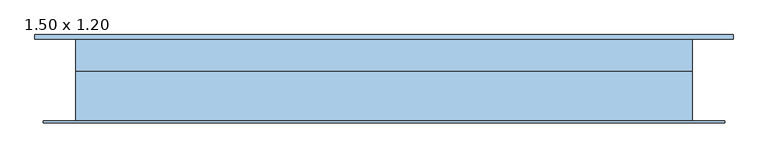
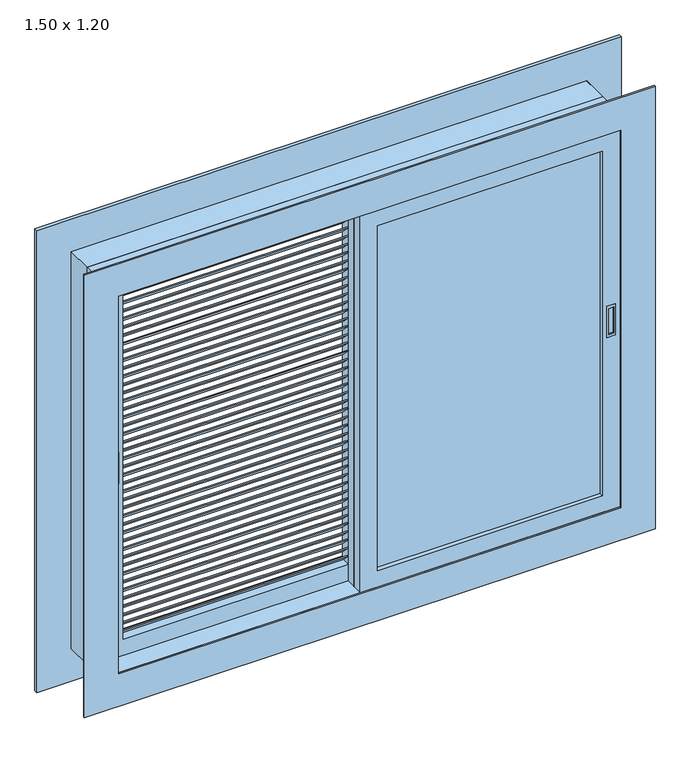
"""IFC4 building model written with IfcOpenShell, lengths in millimetres: window geometry, CC_JANELA CORRER_2 FOLHAS VENEZIANAS + 1 FOLHA VIDRO : 1.50 x 1.20."""

from ifc_helpers import new_model, si_unit, frame, origin, place, context, project, spatial, polyline, outline, extrude, faceted_brep, source, transform, mapped, element, save


def window_1_50_x_1_20_c4f364b7(model_context):
    return source(origin(), model_context, "Body", "SolidModel", [
        extrude(outline(polyline([(-65.0, 2109.7619048), (-40.0, 2084.7619048), (-45.0, 2084.7619048), (-70.0, 2109.7619048), (-65.0, 2109.7619048)])), frame((25.0, 0.0, 0.0), z_axis=(1.0, 0.0, 0.0), x_axis=(0.0, 1.0, 0.0)), (0.0, 0.0, 1.0), 655.0),
        extrude(outline(polyline([(-65.0, 2084.5238095), (-40.0, 2059.5238095), (-45.0, 2059.5238095), (-70.0, 2084.5238095), (-65.0, 2084.5238095)])), frame((25.0, 0.0, 0.0), z_axis=(1.0, 0.0, 0.0), x_axis=(0.0, 1.0, 0.0)), (0.0, 0.0, 1.0), 655.0),
        extrude(outline(polyline([(-65.0, 2059.2857143), (-40.0, 2034.2857143), (-45.0, 2034.2857143), (-70.0, 2059.2857143), (-65.0, 2059.2857143)])), frame((25.0, 0.0, 0.0), z_axis=(1.0, 0.0, 0.0), x_axis=(0.0, 1.0, 0.0)), (0.0, 0.0, 1.0), 655.0),
        extrude(outline(polyline([(-65.0, 2034.047619), (-40.0, 2009.047619), (-45.0, 2009.047619), (-70.0, 2034.047619), (-65.0, 2034.047619)])), frame((25.0, 0.0, 0.0), z_axis=(1.0, 0.0, 0.0), x_axis=(0.0, 1.0, 0.0)), (0.0, 0.0, 1.0), 655.0),
        extrude(outline(polyline([(-65.0, 2008.8095238), (-40.0, 1983.8095238), (-45.0, 1983.8095238), (-70.0, 2008.8095238), (-65.0, 2008.8095238)])), frame((25.0, 0.0, 0.0), z_axis=(1.0, 0.0, 0.0), x_axis=(0.0, 1.0, 0.0)), (0.0, 0.0, 1.0), 655.0),
        extrude(outline(polyline([(-65.0, 1983.5714286), (-40.0, 1958.5714286), (-45.0, 1958.5714286), (-70.0, 1983.5714286), (-65.0, 1983.5714286)])), frame((25.0, 0.0, 0.0), z_axis=(1.0, 0.0, 0.0), x_axis=(0.0, 1.0, 0.0)), (0.0, 0.0, 1.0), 655.0),
        extrude(outline(polyline([(-65.0, 1958.3333333), (-40.0, 1933.3333333), (-45.0, 1933.3333333), (-70.0, 1958.3333333), (-65.0, 1958.3333333)])), frame((25.0, 0.0, 0.0), z_axis=(1.0, 0.0, 0.0), x_axis=(0.0, 1.0, 0.0)), (0.0, 0.0, 1.0), 655.0),
        extrude(outline(polyline([(-65.0, 1933.0952381), (-40.0, 1908.0952381), (-45.0, 1908.0952381), (-70.0, 1933.0952381), (-65.0, 1933.0952381)])), frame((25.0, 0.0, 0.0), z_axis=(1.0, 0.0, 0.0), x_axis=(0.0, 1.0, 0.0)), (0.0, 0.0, 1.0), 655.0),
        extrude(outline(polyline([(-65.0, 1907.8571429), (-40.0, 1882.8571429), (-45.0, 1882.8571429), (-70.0, 1907.8571429), (-65.0, 1907.8571429)])), frame((25.0, 0.0, 0.0), z_axis=(1.0, 0.0, 0.0), x_axis=(0.0, 1.0, 0.0)), (0.0, 0.0, 1.0), 655.0),
        extrude(outline(polyline([(-65.0, 1882.6190476), (-40.0, 1857.6190476), (-45.0, 1857.6190476), (-70.0, 1882.6190476), (-65.0, 1882.6190476)])), frame((25.0, 0.0, 0.0), z_axis=(1.0, 0.0, 0.0), x_axis=(0.0, 1.0, 0.0)), (0.0, 0.0, 1.0), 655.0),
        extrude(outline(polyline([(-65.0, 1857.3809524), (-40.0, 1832.3809524), (-45.0, 1832.3809524), (-70.0, 1857.3809524), (-65.0, 1857.3809524)])), frame((25.0, 0.0, 0.0), z_axis=(1.0, 0.0, 0.0), x_axis=(0.0, 1.0, 0.0)), (0.0, 0.0, 1.0), 655.0),
        extrude(outline(polyline([(-65.0, 1832.1428571), (-40.0, 1807.1428571), (-45.0, 1807.1428571), (-70.0, 1832.1428571), (-65.0, 1832.1428571)])), frame((25.0, 0.0, 0.0), z_axis=(1.0, 0.0, 0.0), x_axis=(0.0, 1.0, 0.0)), (0.0, 0.0, 1.0), 655.0),
        extrude(outline(polyline([(-65.0, 1806.9047619), (-40.0, 1781.9047619), (-45.0, 1781.9047619), (-70.0, 1806.9047619), (-65.0, 1806.9047619)])), frame((25.0, 0.0, 0.0), z_axis=(1.0, 0.0, 0.0), x_axis=(0.0, 1.0, 0.0)), (0.0, 0.0, 1.0), 655.0),
        extrude(outline(polyline([(-65.0, 1781.6666667), (-40.0, 1756.6666667), (-45.0, 1756.6666667), (-70.0, 1781.6666667), (-65.0, 1781.6666667)])), frame((25.0, 0.0, 0.0), z_axis=(1.0, 0.0, 0.0), x_axis=(0.0, 1.0, 0.0)), (0.0, 0.0, 1.0), 655.0),
        extrude(outline(polyline([(-65.0, 1756.4285714), (-40.0, 1731.4285714), (-45.0, 1731.4285714), (-70.0, 1756.4285714), (-65.0, 1756.4285714)])), frame((25.0, 0.0, 0.0), z_axis=(1.0, 0.0, 0.0), x_axis=(0.0, 1.0, 0.0)), (0.0, 0.0, 1.0), 655.0),
        extrude(outline(polyline([(-65.0, 1731.1904762), (-40.0, 1706.1904762), (-45.0, 1706.1904762), (-70.0, 1731.1904762), (-65.0, 1731.1904762)])), frame((25.0, 0.0, 0.0), z_axis=(1.0, 0.0, 0.0), x_axis=(0.0, 1.0, 0.0)), (0.0, 0.0, 1.0), 655.0),
        extrude(outline(polyline([(-65.0, 1705.952381), (-40.0, 1680.952381), (-45.0, 1680.952381), (-70.0, 1705.952381), (-65.0, 1705.952381)])), frame((25.0, 0.0, 0.0), z_axis=(1.0, 0.0, 0.0), x_axis=(0.0, 1.0, 0.0)), (0.0, 0.0, 1.0), 655.0),
        extrude(outline(polyline([(-65.0, 1680.7142857), (-40.0, 1655.7142857), (-45.0, 1655.7142857), (-70.0, 1680.7142857), (-65.0, 1680.7142857)])), frame((25.0, 0.0, 0.0), z_axis=(1.0, 0.0, 0.0), x_axis=(0.0, 1.0, 0.0)), (0.0, 0.0, 1.0), 655.0),
        extrude(outline(polyline([(-65.0, 1655.4761905), (-40.0, 1630.4761905), (-45.0, 1630.4761905), (-70.0, 1655.4761905), (-65.0, 1655.4761905)])), frame((25.0, 0.0, 0.0), z_axis=(1.0, 0.0, 0.0), x_axis=(0.0, 1.0, 0.0)), (0.0, 0.0, 1.0), 655.0),
        extrude(outline(polyline([(-65.0, 1630.2380952), (-40.0, 1605.2380952), (-45.0, 1605.2380952), (-70.0, 1630.2380952), (-65.0, 1630.2380952)])), frame((25.0, 0.0, 0.0), z_axis=(1.0, 0.0, 0.0), x_axis=(0.0, 1.0, 0.0)), (0.0, 0.0, 1.0), 655.0),
        extrude(outline(polyline([(-65.0, 1605.0), (-40.0, 1580.0), (-45.0, 1580.0), (-70.0, 1605.0), (-65.0, 1605.0)])), frame((25.0, 0.0, 0.0), z_axis=(1.0, 0.0, 0.0), x_axis=(0.0, 1.0, 0.0)), (0.0, 0.0, 1.0), 655.0),
        extrude(outline(polyline([(-65.0, 1579.7619048), (-40.0, 1554.7619048), (-45.0, 1554.7619048), (-70.0, 1579.7619048), (-65.0, 1579.7619048)])), frame((25.0, 0.0, 0.0), z_axis=(1.0, 0.0, 0.0), x_axis=(0.0, 1.0, 0.0)), (0.0, 0.0, 1.0), 655.0),
        extrude(outline(polyline([(-65.0, 1554.5238095), (-40.0, 1529.5238095), (-45.0, 1529.5238095), (-70.0, 1554.5238095), (-65.0, 1554.5238095)])), frame((25.0, 0.0, 0.0), z_axis=(1.0, 0.0, 0.0), x_axis=(0.0, 1.0, 0.0)), (0.0, 0.0, 1.0), 655.0),
        extrude(outline(polyline([(-65.0, 1529.2857143), (-40.0, 1504.2857143), (-45.0, 1504.2857143), (-70.0, 1529.2857143), (-65.0, 1529.2857143)])), frame((25.0, 0.0, 0.0), z_axis=(1.0, 0.0, 0.0), x_axis=(0.0, 1.0, 0.0)), (0.0, 0.0, 1.0), 655.0),
        extrude(outline(polyline([(-65.0, 1504.047619), (-40.0, 1479.047619), (-45.0, 1479.047619), (-70.0, 1504.047619), (-65.0, 1504.047619)])), frame((25.0, 0.0, 0.0), z_axis=(1.0, 0.0, 0.0), x_axis=(0.0, 1.0, 0.0)), (0.0, 0.0, 1.0), 655.0),
        extrude(outline(polyline([(-65.0, 1478.8095238), (-40.0, 1453.8095238), (-45.0, 1453.8095238), (-70.0, 1478.8095238), (-65.0, 1478.8095238)])), frame((25.0, 0.0, 0.0), z_axis=(1.0, 0.0, 0.0), x_axis=(0.0, 1.0, 0.0)), (0.0, 0.0, 1.0), 655.0),
        extrude(outline(polyline([(-65.0, 1453.5714286), (-40.0, 1428.5714286), (-45.0, 1428.5714286), (-70.0, 1453.5714286), (-65.0, 1453.5714286)])), frame((25.0, 0.0, 0.0), z_axis=(1.0, 0.0, 0.0), x_axis=(0.0, 1.0, 0.0)), (0.0, 0.0, 1.0), 655.0),
        extrude(outline(polyline([(-65.0, 1428.3333333), (-40.0, 1403.3333333), (-45.0, 1403.3333333), (-70.0, 1428.3333333), (-65.0, 1428.3333333)])), frame((25.0, 0.0, 0.0), z_axis=(1.0, 0.0, 0.0), x_axis=(0.0, 1.0, 0.0)), (0.0, 0.0, 1.0), 655.0),
        extrude(outline(polyline([(-65.0, 1403.0952381), (-40.0, 1378.0952381), (-45.0, 1378.0952381), (-70.0, 1403.0952381), (-65.0, 1403.0952381)])), frame((25.0, 0.0, 0.0), z_axis=(1.0, 0.0, 0.0), x_axis=(0.0, 1.0, 0.0)), (0.0, 0.0, 1.0), 655.0),
        extrude(outline(polyline([(-65.0, 1377.8571429), (-40.0, 1352.8571429), (-45.0, 1352.8571429), (-70.0, 1377.8571429), (-65.0, 1377.8571429)])), frame((25.0, 0.0, 0.0), z_axis=(1.0, 0.0, 0.0), x_axis=(0.0, 1.0, 0.0)), (0.0, 0.0, 1.0), 655.0),
        extrude(outline(polyline([(-65.0, 1352.6190476), (-40.0, 1327.6190476), (-45.0, 1327.6190476), (-70.0, 1352.6190476), (-65.0, 1352.6190476)])), frame((25.0, 0.0, 0.0), z_axis=(1.0, 0.0, 0.0), x_axis=(0.0, 1.0, 0.0)), (0.0, 0.0, 1.0), 655.0),
        extrude(outline(polyline([(-65.0, 1327.3809524), (-40.0, 1302.3809524), (-45.0, 1302.3809524), (-70.0, 1327.3809524), (-65.0, 1327.3809524)])), frame((25.0, 0.0, 0.0), z_axis=(1.0, 0.0, 0.0), x_axis=(0.0, 1.0, 0.0)), (0.0, 0.0, 1.0), 655.0),
        extrude(outline(polyline([(-65.0, 1302.1428571), (-40.0, 1277.1428571), (-45.0, 1277.1428571), (-70.0, 1302.1428571), (-65.0, 1302.1428571)])), frame((25.0, 0.0, 0.0), z_axis=(1.0, 0.0, 0.0), x_axis=(0.0, 1.0, 0.0)), (0.0, 0.0, 1.0), 655.0),
        extrude(outline(polyline([(-65.0, 1276.9047619), (-40.0, 1251.9047619), (-45.0, 1251.9047619), (-70.0, 1276.9047619), (-65.0, 1276.9047619)])), frame((25.0, 0.0, 0.0), z_axis=(1.0, 0.0, 0.0), x_axis=(0.0, 1.0, 0.0)), (0.0, 0.0, 1.0), 655.0),
        extrude(outline(polyline([(-65.0, 1251.6666667), (-40.0, 1226.6666667), (-45.0, 1226.6666667), (-70.0, 1251.6666667), (-65.0, 1251.6666667)])), frame((25.0, 0.0, 0.0), z_axis=(1.0, 0.0, 0.0), x_axis=(0.0, 1.0, 0.0)), (0.0, 0.0, 1.0), 655.0),
        extrude(outline(polyline([(-65.0, 1226.4285714), (-40.0, 1201.4285714), (-45.0, 1201.4285714), (-70.0, 1226.4285714), (-65.0, 1226.4285714)])), frame((25.0, 0.0, 0.0), z_axis=(1.0, 0.0, 0.0), x_axis=(0.0, 1.0, 0.0)), (0.0, 0.0, 1.0), 655.0),
        extrude(outline(polyline([(-65.0, 1201.1904762), (-40.0, 1176.1904762), (-45.0, 1176.1904762), (-70.0, 1201.1904762), (-65.0, 1201.1904762)])), frame((25.0, 0.0, 0.0), z_axis=(1.0, 0.0, 0.0), x_axis=(0.0, 1.0, 0.0)), (0.0, 0.0, 1.0), 655.0),
        extrude(outline(polyline([(-65.0, 1175.952381), (-40.0, 1150.952381), (-45.0, 1150.952381), (-70.0, 1175.952381), (-65.0, 1175.952381)])), frame((25.0, 0.0, 0.0), z_axis=(1.0, 0.0, 0.0), x_axis=(0.0, 1.0, 0.0)), (0.0, 0.0, 1.0), 655.0),
        extrude(outline(polyline([(-65.0, 1150.7142857), (-40.0, 1125.7142857), (-45.0, 1125.7142857), (-70.0, 1150.7142857), (-65.0, 1150.7142857)])), frame((25.0, 0.0, 0.0), z_axis=(1.0, 0.0, 0.0), x_axis=(0.0, 1.0, 0.0)), (0.0, 0.0, 1.0), 655.0),
        extrude(outline(polyline([(-65.0, 1125.4761905), (-40.0, 1100.4761905), (-45.0, 1100.4761905), (-70.0, 1125.4761905), (-65.0, 1125.4761905)])), frame((25.0, 0.0, 0.0), z_axis=(1.0, 0.0, 0.0), x_axis=(0.0, 1.0, 0.0)), (0.0, 0.0, 1.0), 655.0),
        extrude(outline(polyline([(-65.0, 1100.2380952), (-40.0, 1075.2380952), (-45.0, 1075.2380952), (-70.0, 1100.2380952), (-65.0, 1100.2380952)])), frame((25.0, 0.0, 0.0), z_axis=(1.0, 0.0, 0.0), x_axis=(0.0, 1.0, 0.0)), (0.0, 0.0, 1.0), 655.0),
        extrude(outline(polyline([(697.5, -66.0), (697.5, -65.0), (712.5, -65.0), (712.5, -66.0), (697.5, -66.0)])), frame((0.0, 0.0, 1540.0), z_axis=(0.0, 0.0, 1.0), x_axis=(1.0, 0.0, 0.0)), (0.0, 0.0, 1.0), 80.0),
        extrude(outline(polyline([(1532.0, 717.5), (1628.0, 717.5), (1628.0, 692.5), (1532.0, 692.5), (1532.0, 717.5)]), holes=[polyline([(1540.0, 712.5), (1540.0, 697.5), (1620.0, 697.5), (1620.0, 712.5), (1540.0, 712.5)])]), frame((0.0, -70.1, 0.0), z_axis=(0.0, 1.0, 0.0), x_axis=(0.0, 0.0, 1.0)), (0.0, 0.0, 1.0), 5.1),
        extrude(outline(polyline([(-65.0, 1075.0), (-40.0, 1050.0), (-45.0, 1050.0), (-70.0, 1075.0), (-65.0, 1075.0)])), frame((25.0, 0.0, 0.0), z_axis=(1.0, 0.0, 0.0), x_axis=(0.0, 1.0, 0.0)), (0.0, 0.0, 1.0), 655.0),
        extrude(outline(polyline([(2160.0, 730.0), (2160.0, -25.0), (1000.0, -25.0), (1000.0, 730.0), (2160.0, 730.0)]), holes=[polyline([(2110.0, 25.0), (2110.0, 680.0), (1050.0, 680.0), (1050.0, 25.0), (2110.0, 25.0)])]), frame((0.0, -70.0, 0.0), z_axis=(0.0, 1.0, 0.0), x_axis=(0.0, 0.0, 1.0)), (0.0, 0.0, 1.0), 30.0),
        extrude(outline(polyline([(-35.0, 2109.7619048), (-10.0, 2084.7619048), (-15.0, 2084.7619048), (-40.0, 2109.7619048), (-35.0, 2109.7619048)])), frame((-680.0, 0.0, 0.0), z_axis=(1.0, 0.0, 0.0), x_axis=(0.0, 1.0, 0.0)), (0.0, 0.0, 1.0), 655.0),
        extrude(outline(polyline([(-35.0, 2084.5238095), (-10.0, 2059.5238095), (-15.0, 2059.5238095), (-40.0, 2084.5238095), (-35.0, 2084.5238095)])), frame((-680.0, 0.0, 0.0), z_axis=(1.0, 0.0, 0.0), x_axis=(0.0, 1.0, 0.0)), (0.0, 0.0, 1.0), 655.0),
        extrude(outline(polyline([(-35.0, 2059.2857143), (-10.0, 2034.2857143), (-15.0, 2034.2857143), (-40.0, 2059.2857143), (-35.0, 2059.2857143)])), frame((-680.0, 0.0, 0.0), z_axis=(1.0, 0.0, 0.0), x_axis=(0.0, 1.0, 0.0)), (0.0, 0.0, 1.0), 655.0),
        extrude(outline(polyline([(-35.0, 2034.047619), (-10.0, 2009.047619), (-15.0, 2009.047619), (-40.0, 2034.047619), (-35.0, 2034.047619)])), frame((-680.0, 0.0, 0.0), z_axis=(1.0, 0.0, 0.0), x_axis=(0.0, 1.0, 0.0)), (0.0, 0.0, 1.0), 655.0),
        extrude(outline(polyline([(-35.0, 2008.8095238), (-10.0, 1983.8095238), (-15.0, 1983.8095238), (-40.0, 2008.8095238), (-35.0, 2008.8095238)])), frame((-680.0, 0.0, 0.0), z_axis=(1.0, 0.0, 0.0), x_axis=(0.0, 1.0, 0.0)), (0.0, 0.0, 1.0), 655.0),
        extrude(outline(polyline([(-35.0, 1983.5714286), (-10.0, 1958.5714286), (-15.0, 1958.5714286), (-40.0, 1983.5714286), (-35.0, 1983.5714286)])), frame((-680.0, 0.0, 0.0), z_axis=(1.0, 0.0, 0.0), x_axis=(0.0, 1.0, 0.0)), (0.0, 0.0, 1.0), 655.0),
        extrude(outline(polyline([(-35.0, 1958.3333333), (-10.0, 1933.3333333), (-15.0, 1933.3333333), (-40.0, 1958.3333333), (-35.0, 1958.3333333)])), frame((-680.0, 0.0, 0.0), z_axis=(1.0, 0.0, 0.0), x_axis=(0.0, 1.0, 0.0)), (0.0, 0.0, 1.0), 655.0),
        extrude(outline(polyline([(-35.0, 1933.0952381), (-10.0, 1908.0952381), (-15.0, 1908.0952381), (-40.0, 1933.0952381), (-35.0, 1933.0952381)])), frame((-680.0, 0.0, 0.0), z_axis=(1.0, 0.0, 0.0), x_axis=(0.0, 1.0, 0.0)), (0.0, 0.0, 1.0), 655.0),
        extrude(outline(polyline([(-35.0, 1907.8571429), (-10.0, 1882.8571429), (-15.0, 1882.8571429), (-40.0, 1907.8571429), (-35.0, 1907.8571429)])), frame((-680.0, 0.0, 0.0), z_axis=(1.0, 0.0, 0.0), x_axis=(0.0, 1.0, 0.0)), (0.0, 0.0, 1.0), 655.0),
        extrude(outline(polyline([(-35.0, 1882.6190476), (-10.0, 1857.6190476), (-15.0, 1857.6190476), (-40.0, 1882.6190476), (-35.0, 1882.6190476)])), frame((-680.0, 0.0, 0.0), z_axis=(1.0, 0.0, 0.0), x_axis=(0.0, 1.0, 0.0)), (0.0, 0.0, 1.0), 655.0),
        extrude(outline(polyline([(-35.0, 1857.3809524), (-10.0, 1832.3809524), (-15.0, 1832.3809524), (-40.0, 1857.3809524), (-35.0, 1857.3809524)])), frame((-680.0, 0.0, 0.0), z_axis=(1.0, 0.0, 0.0), x_axis=(0.0, 1.0, 0.0)), (0.0, 0.0, 1.0), 655.0),
        extrude(outline(polyline([(-35.0, 1832.1428571), (-10.0, 1807.1428571), (-15.0, 1807.1428571), (-40.0, 1832.1428571), (-35.0, 1832.1428571)])), frame((-680.0, 0.0, 0.0), z_axis=(1.0, 0.0, 0.0), x_axis=(0.0, 1.0, 0.0)), (0.0, 0.0, 1.0), 655.0),
        extrude(outline(polyline([(-35.0, 1806.9047619), (-10.0, 1781.9047619), (-15.0, 1781.9047619), (-40.0, 1806.9047619), (-35.0, 1806.9047619)])), frame((-680.0, 0.0, 0.0), z_axis=(1.0, 0.0, 0.0), x_axis=(0.0, 1.0, 0.0)), (0.0, 0.0, 1.0), 655.0),
        extrude(outline(polyline([(-35.0, 1781.6666667), (-10.0, 1756.6666667), (-15.0, 1756.6666667), (-40.0, 1781.6666667), (-35.0, 1781.6666667)])), frame((-680.0, 0.0, 0.0), z_axis=(1.0, 0.0, 0.0), x_axis=(0.0, 1.0, 0.0)), (0.0, 0.0, 1.0), 655.0),
        extrude(outline(polyline([(-35.0, 1756.4285714), (-10.0, 1731.4285714), (-15.0, 1731.4285714), (-40.0, 1756.4285714), (-35.0, 1756.4285714)])), frame((-680.0, 0.0, 0.0), z_axis=(1.0, 0.0, 0.0), x_axis=(0.0, 1.0, 0.0)), (0.0, 0.0, 1.0), 655.0),
        extrude(outline(polyline([(-35.0, 1731.1904762), (-10.0, 1706.1904762), (-15.0, 1706.1904762), (-40.0, 1731.1904762), (-35.0, 1731.1904762)])), frame((-680.0, 0.0, 0.0), z_axis=(1.0, 0.0, 0.0), x_axis=(0.0, 1.0, 0.0)), (0.0, 0.0, 1.0), 655.0),
        extrude(outline(polyline([(-35.0, 1705.952381), (-10.0, 1680.952381), (-15.0, 1680.952381), (-40.0, 1705.952381), (-35.0, 1705.952381)])), frame((-680.0, 0.0, 0.0), z_axis=(1.0, 0.0, 0.0), x_axis=(0.0, 1.0, 0.0)), (0.0, 0.0, 1.0), 655.0),
        extrude(outline(polyline([(-35.0, 1680.7142857), (-10.0, 1655.7142857), (-15.0, 1655.7142857), (-40.0, 1680.7142857), (-35.0, 1680.7142857)])), frame((-680.0, 0.0, 0.0), z_axis=(1.0, 0.0, 0.0), x_axis=(0.0, 1.0, 0.0)), (0.0, 0.0, 1.0), 655.0),
        extrude(outline(polyline([(-35.0, 1655.4761905), (-10.0, 1630.4761905), (-15.0, 1630.4761905), (-40.0, 1655.4761905), (-35.0, 1655.4761905)])), frame((-680.0, 0.0, 0.0), z_axis=(1.0, 0.0, 0.0), x_axis=(0.0, 1.0, 0.0)), (0.0, 0.0, 1.0), 655.0),
        extrude(outline(polyline([(-35.0, 1630.2380952), (-10.0, 1605.2380952), (-15.0, 1605.2380952), (-40.0, 1630.2380952), (-35.0, 1630.2380952)])), frame((-680.0, 0.0, 0.0), z_axis=(1.0, 0.0, 0.0), x_axis=(0.0, 1.0, 0.0)), (0.0, 0.0, 1.0), 655.0),
        extrude(outline(polyline([(-35.0, 1605.0), (-10.0, 1580.0), (-15.0, 1580.0), (-40.0, 1605.0), (-35.0, 1605.0)])), frame((-680.0, 0.0, 0.0), z_axis=(1.0, 0.0, 0.0), x_axis=(0.0, 1.0, 0.0)), (0.0, 0.0, 1.0), 655.0),
        extrude(outline(polyline([(-35.0, 1579.7619048), (-10.0, 1554.7619048), (-15.0, 1554.7619048), (-40.0, 1579.7619048), (-35.0, 1579.7619048)])), frame((-680.0, 0.0, 0.0), z_axis=(1.0, 0.0, 0.0), x_axis=(0.0, 1.0, 0.0)), (0.0, 0.0, 1.0), 655.0),
        extrude(outline(polyline([(-35.0, 1554.5238095), (-10.0, 1529.5238095), (-15.0, 1529.5238095), (-40.0, 1554.5238095), (-35.0, 1554.5238095)])), frame((-680.0, 0.0, 0.0), z_axis=(1.0, 0.0, 0.0), x_axis=(0.0, 1.0, 0.0)), (0.0, 0.0, 1.0), 655.0),
        extrude(outline(polyline([(-35.0, 1529.2857143), (-10.0, 1504.2857143), (-15.0, 1504.2857143), (-40.0, 1529.2857143), (-35.0, 1529.2857143)])), frame((-680.0, 0.0, 0.0), z_axis=(1.0, 0.0, 0.0), x_axis=(0.0, 1.0, 0.0)), (0.0, 0.0, 1.0), 655.0),
        extrude(outline(polyline([(-35.0, 1504.047619), (-10.0, 1479.047619), (-15.0, 1479.047619), (-40.0, 1504.047619), (-35.0, 1504.047619)])), frame((-680.0, 0.0, 0.0), z_axis=(1.0, 0.0, 0.0), x_axis=(0.0, 1.0, 0.0)), (0.0, 0.0, 1.0), 655.0),
        extrude(outline(polyline([(-35.0, 1478.8095238), (-10.0, 1453.8095238), (-15.0, 1453.8095238), (-40.0, 1478.8095238), (-35.0, 1478.8095238)])), frame((-680.0, 0.0, 0.0), z_axis=(1.0, 0.0, 0.0), x_axis=(0.0, 1.0, 0.0)), (0.0, 0.0, 1.0), 655.0),
        extrude(outline(polyline([(-35.0, 1453.5714286), (-10.0, 1428.5714286), (-15.0, 1428.5714286), (-40.0, 1453.5714286), (-35.0, 1453.5714286)])), frame((-680.0, 0.0, 0.0), z_axis=(1.0, 0.0, 0.0), x_axis=(0.0, 1.0, 0.0)), (0.0, 0.0, 1.0), 655.0),
        extrude(outline(polyline([(-35.0, 1428.3333333), (-10.0, 1403.3333333), (-15.0, 1403.3333333), (-40.0, 1428.3333333), (-35.0, 1428.3333333)])), frame((-680.0, 0.0, 0.0), z_axis=(1.0, 0.0, 0.0), x_axis=(0.0, 1.0, 0.0)), (0.0, 0.0, 1.0), 655.0),
        extrude(outline(polyline([(-35.0, 1403.0952381), (-10.0, 1378.0952381), (-15.0, 1378.0952381), (-40.0, 1403.0952381), (-35.0, 1403.0952381)])), frame((-680.0, 0.0, 0.0), z_axis=(1.0, 0.0, 0.0), x_axis=(0.0, 1.0, 0.0)), (0.0, 0.0, 1.0), 655.0),
        extrude(outline(polyline([(-35.0, 1377.8571429), (-10.0, 1352.8571429), (-15.0, 1352.8571429), (-40.0, 1377.8571429), (-35.0, 1377.8571429)])), frame((-680.0, 0.0, 0.0), z_axis=(1.0, 0.0, 0.0), x_axis=(0.0, 1.0, 0.0)), (0.0, 0.0, 1.0), 655.0),
        extrude(outline(polyline([(-35.0, 1352.6190476), (-10.0, 1327.6190476), (-15.0, 1327.6190476), (-40.0, 1352.6190476), (-35.0, 1352.6190476)])), frame((-680.0, 0.0, 0.0), z_axis=(1.0, 0.0, 0.0), x_axis=(0.0, 1.0, 0.0)), (0.0, 0.0, 1.0), 655.0),
        extrude(outline(polyline([(-35.0, 1327.3809524), (-10.0, 1302.3809524), (-15.0, 1302.3809524), (-40.0, 1327.3809524), (-35.0, 1327.3809524)])), frame((-680.0, 0.0, 0.0), z_axis=(1.0, 0.0, 0.0), x_axis=(0.0, 1.0, 0.0)), (0.0, 0.0, 1.0), 655.0),
        extrude(outline(polyline([(-35.0, 1302.1428571), (-10.0, 1277.1428571), (-15.0, 1277.1428571), (-40.0, 1302.1428571), (-35.0, 1302.1428571)])), frame((-680.0, 0.0, 0.0), z_axis=(1.0, 0.0, 0.0), x_axis=(0.0, 1.0, 0.0)), (0.0, 0.0, 1.0), 655.0),
        extrude(outline(polyline([(-35.0, 1276.9047619), (-10.0, 1251.9047619), (-15.0, 1251.9047619), (-40.0, 1276.9047619), (-35.0, 1276.9047619)])), frame((-680.0, 0.0, 0.0), z_axis=(1.0, 0.0, 0.0), x_axis=(0.0, 1.0, 0.0)), (0.0, 0.0, 1.0), 655.0),
        extrude(outline(polyline([(-35.0, 1251.6666667), (-10.0, 1226.6666667), (-15.0, 1226.6666667), (-40.0, 1251.6666667), (-35.0, 1251.6666667)])), frame((-680.0, 0.0, 0.0), z_axis=(1.0, 0.0, 0.0), x_axis=(0.0, 1.0, 0.0)), (0.0, 0.0, 1.0), 655.0),
        extrude(outline(polyline([(-35.0, 1226.4285714), (-10.0, 1201.4285714), (-15.0, 1201.4285714), (-40.0, 1226.4285714), (-35.0, 1226.4285714)])), frame((-680.0, 0.0, 0.0), z_axis=(1.0, 0.0, 0.0), x_axis=(0.0, 1.0, 0.0)), (0.0, 0.0, 1.0), 655.0),
        extrude(outline(polyline([(-35.0, 1201.1904762), (-10.0, 1176.1904762), (-15.0, 1176.1904762), (-40.0, 1201.1904762), (-35.0, 1201.1904762)])), frame((-680.0, 0.0, 0.0), z_axis=(1.0, 0.0, 0.0), x_axis=(0.0, 1.0, 0.0)), (0.0, 0.0, 1.0), 655.0),
        extrude(outline(polyline([(-35.0, 1175.952381), (-10.0, 1150.952381), (-15.0, 1150.952381), (-40.0, 1175.952381), (-35.0, 1175.952381)])), frame((-680.0, 0.0, 0.0), z_axis=(1.0, 0.0, 0.0), x_axis=(0.0, 1.0, 0.0)), (0.0, 0.0, 1.0), 655.0),
        extrude(outline(polyline([(-35.0, 1150.7142857), (-10.0, 1125.7142857), (-15.0, 1125.7142857), (-40.0, 1150.7142857), (-35.0, 1150.7142857)])), frame((-680.0, 0.0, 0.0), z_axis=(1.0, 0.0, 0.0), x_axis=(0.0, 1.0, 0.0)), (0.0, 0.0, 1.0), 655.0),
        extrude(outline(polyline([(-35.0, 1125.4761905), (-10.0, 1100.4761905), (-15.0, 1100.4761905), (-40.0, 1125.4761905), (-35.0, 1125.4761905)])), frame((-680.0, 0.0, 0.0), z_axis=(1.0, 0.0, 0.0), x_axis=(0.0, 1.0, 0.0)), (0.0, 0.0, 1.0), 655.0),
        extrude(outline(polyline([(-35.0, 1100.2380952), (-10.0, 1075.2380952), (-15.0, 1075.2380952), (-40.0, 1100.2380952), (-35.0, 1100.2380952)])), frame((-680.0, 0.0, 0.0), z_axis=(1.0, 0.0, 0.0), x_axis=(0.0, 1.0, 0.0)), (0.0, 0.0, 1.0), 655.0),
        extrude(outline(polyline([(-697.5, -36.0), (-712.5, -36.0), (-712.5, -35.0), (-697.5, -35.0), (-697.5, -36.0)])), frame((0.0, 0.0, 1540.0), z_axis=(0.0, 0.0, 1.0), x_axis=(1.0, 0.0, 0.0)), (0.0, 0.0, 1.0), 80.0),
        extrude(outline(polyline([(1532.0, -717.5), (1532.0, -692.5), (1628.0, -692.5), (1628.0, -717.5), (1532.0, -717.5)]), holes=[polyline([(1540.0, -712.5), (1620.0, -712.5), (1620.0, -697.5), (1540.0, -697.5), (1540.0, -712.5)])]), frame((0.0, -40.1, 0.0), z_axis=(0.0, 1.0, 0.0), x_axis=(0.0, 0.0, 1.0)), (0.0, 0.0, 1.0), 5.1),
        extrude(outline(polyline([(-35.0, 1075.0), (-10.0, 1050.0), (-15.0, 1050.0), (-40.0, 1075.0), (-35.0, 1075.0)])), frame((-680.0, 0.0, 0.0), z_axis=(1.0, 0.0, 0.0), x_axis=(0.0, 1.0, 0.0)), (0.0, 0.0, 1.0), 655.0),
        extrude(outline(polyline([(2160.0, -730.0), (1000.0, -730.0), (1000.0, 25.0), (2160.0, 25.0), (2160.0, -730.0)]), holes=[polyline([(2110.0, -25.0), (1050.0, -25.0), (1050.0, -680.0), (2110.0, -680.0), (2110.0, -25.0)])]), frame((0.0, -40.0, 0.0), z_axis=(0.0, 1.0, 0.0), x_axis=(0.0, 0.0, 1.0)), (0.0, 0.0, 1.0), 30.0),
        extrude(outline(polyline([(712.5, -96.0), (697.5, -96.0), (697.5, -95.0), (712.5, -95.0), (712.5, -96.0)])), frame((0.0, 0.0, 1540.0), z_axis=(0.0, 0.0, 1.0), x_axis=(1.0, 0.0, 0.0)), (0.0, 0.0, 1.0), 80.0),
        extrude(outline(polyline([(1532.0, 692.5), (1532.0, 717.5), (1628.0, 717.5), (1628.0, 692.5), (1532.0, 692.5)]), holes=[polyline([(1540.0, 697.5), (1620.0, 697.5), (1620.0, 712.5), (1540.0, 712.5), (1540.0, 697.5)])]), frame((0.0, -100.1, 0.0), z_axis=(0.0, 1.0, 0.0), x_axis=(0.0, 0.0, 1.0)), (0.0, 0.0, 1.0), 5.1),
        faceted_brep([(680.0, -100.0, 2110.0), (680.0, -70.0, 2110.0), (680.0, -70.0, 1050.0), (680.0, -100.0, 1050.0), (730.0, -70.0, 2160.0), (730.0, -100.0, 2160.0), (730.0, -100.0, 1000.0), (730.0, -70.0, 1000.0), (25.0, -70.0, 1050.0), (25.0, -100.0, 1050.0), (-25.0, -100.0, 1000.0), (-25.0, -70.0, 1000.0), (25.0, -70.0, 2110.0), (25.0, -100.0, 2110.0), (-25.0, -100.0, 2160.0), (-25.0, -70.0, 2160.0), (692.5, -100.0, 1628.0), (717.5, -100.0, 1628.0), (717.5, -100.0, 1532.0), (692.5, -100.0, 1532.0), (717.5, -95.0, 1628.0), (692.5, -95.0, 1628.0), (717.5, -95.0, 1532.0), (692.5, -95.0, 1532.0)], [[[0, 1, 2, 3]], [[4, 5, 6, 7]], [[3, 2, 8, 9]], [[7, 6, 10, 11]], [[9, 8, 12, 13]], [[11, 10, 14, 15]], [[4, 7, 11, 15], [2, 1, 12, 8]], [[1, 0, 13, 12]], [[6, 5, 14, 10], [0, 3, 9, 13], [16, 17, 18, 19]], [[5, 4, 15, 14]], [[20, 17, 16, 21]], [[22, 23, 19, 18]], [[20, 21, 23, 22]], [[21, 16, 19, 23]], [[17, 20, 22, 18]]]),
        extrude(outline(polyline([(680.0, -82.5), (680.0, -87.5), (25.0, -87.5), (25.0, -82.5), (680.0, -82.5)])), frame((0.0, 0.0, 1050.0), z_axis=(0.0, 0.0, 1.0), x_axis=(1.0, 0.0, 0.0)), (0.0, 0.0, 1.0), 1060.0),
        extrude(outline(polyline([(2180.0, 750.0), (2180.0, -750.0), (980.0, -750.0), (980.0, 750.0), (2180.0, 750.0)]), holes=[polyline([(2160.0, 730.0), (1000.0, 730.0), (1000.0, -730.0), (2160.0, -730.0), (2160.0, 730.0)])]), frame((0.0, -100.0, 0.0), z_axis=(0.0, 1.0, 0.0), x_axis=(0.0, 0.0, 1.0)), (0.0, 0.0, 1.0), 120.0),
        faceted_brep([(-750.0, 20.0, 2180.0), (-750.0, 100.0, 2180.0), (-750.0, 100.0, 960.0), (-750.0, 20.0, 960.0), (750.0, 100.0, 960.0), (750.0, 20.0, 960.0), (850.0, 100.0, 860.0), (850.0, 100.0, 2280.0), (-850.0, 100.0, 2280.0), (-850.0, 100.0, 860.0), (750.0, 100.0, 2180.0), (750.0, 20.0, 2180.0), (-749.0, 20.0, 961.0), (-749.0, 20.0, 2179.0), (749.0, 20.0, 2179.0), (749.0, 20.0, 961.0), (-749.0, 110.0, 2179.0), (-749.0, 110.0, 961.0), (749.0, 110.0, 961.0), (749.0, 110.0, 2179.0), (-850.0, 110.0, 860.0), (-850.0, 110.0, 2280.0), (850.0, 110.0, 2280.0), (850.0, 110.0, 860.0)], [[[0, 1, 2, 3]], [[3, 2, 4, 5]], [[6, 7, 8, 9], [2, 1, 10, 4]], [[5, 4, 10, 11]], [[5, 11, 0, 3], [12, 13, 14, 15]], [[16, 13, 12, 17]], [[17, 12, 15, 18]], [[18, 15, 14, 19]], [[20, 21, 22, 23], [18, 19, 16, 17]], [[8, 21, 20, 9]], [[9, 20, 23, 6]], [[6, 23, 22, 7]], [[11, 10, 1, 0]], [[19, 14, 13, 16]], [[7, 22, 21, 8]]]),
        extrude(outline(polyline([(2260.0, -830.0), (900.0, -830.0), (900.0, 830.0), (2260.0, 830.0), (2260.0, -830.0)]), holes=[polyline([(2160.0, 730.0), (1000.0, 730.0), (1000.0, -730.0), (2160.0, -730.0), (2160.0, 730.0)])]), frame((0.0, -105.0, 0.0), z_axis=(0.0, 1.0, 0.0), x_axis=(0.0, 0.0, 1.0)), (0.0, 0.0, 1.0), 5.0),
    ])


if __name__ == "__main__":
    model = new_model("IFC4")
    model_context = context("Model", 3, world=origin())
    ifc_project = project(units=[si_unit("LENGTHUNIT", "METRE", prefix="MILLI")], contexts=[model_context])
    site = spatial("IfcSite", under=ifc_project)
    building = spatial("IfcBuilding", under=site)
    placement = place(None, origin())
    window_1_50_x_1_20_shape = window_1_50_x_1_20_c4f364b7(model_context)
    element("IfcWindow", 1, ObjectType="CC_JANELA CORRER_2 FOLHAS VENEZIANAS + 1 FOLHA VIDRO : 1.50 x 1.20", at=placement, inside=building, context=model_context, shape_type="MappedRepresentation", body=[
        mapped(window_1_50_x_1_20_shape, transform((0.0, 0.0, 0.0), x_axis=(1.0, 0.0, 0.0), y_axis=(0.0, 1.0, 0.0), z_axis=(0.0, 0.0, 1.0))),
    ])
    save(model, "model.ifc")

# Revit data of these elements
# Type "CC_JANELA CORRER_2 FOLHAS VENEZIANAS + 1 FOLHA VIDRO : 1.50 x 1.20"
#   Description = "JANELA CORRER 2 FOLHAS VENEZIANAS + 1 FOLHA VIDRO"
#   Type Mark = "J1"
#   Site = "www.construir.arq.br"
#   Empresa = "Cursos Construir"
#   Criado Por = "Roberto Netto"
#   Analytic Construction = "<Nenhum>"
#   Largura Moldura Folha [instance default] = 0.05 m
#   Largura Guarnição Interna [instance default] = 0.10 m
#   Largura Moldura Externa [instance default] = 0.10 m
#   Largura Folha [instance default] = 0.755 m
#   Interna [instance default] = 0.00 m
#   Externa [instance default] = 0.00 m
#   Extensão Frontal Peitoril/Pingadeira [instance default] = 0.03 m
#   Extensão Exterior Esquerda Peitoril/Pingadeira [instance default] = 0.025 m
#   Extensão Exterior Direita Peitoril/Pingadeira [instance default] = 0.025 m
#   Extensão Caixilho [instance default] = 0.03 m
#   Espessura Peitoril/Pingadeira [instance default] = 0.02 m
#   Espessura Guarnição Interna [instance default] = 0.005 m
#   Espessura Moldura Externa [instance default] = 0.01 m
#   Espessura Folha [instance default] = 0.03 m
#   Cálculo Abertura Vidro [instance default] = 0.00 m
#   Espessura Caixilho [instance default] = 0.02 m
#   Cálculo Abertura Veneziana [instance default] = 0.00 m
#   Altura Folha [instance default] = 1.16 m
#   Altura Palheta Veneziana [instance default] = 0.025 m
#   Altura Corte [instance default] = 0.02 m
#   Height = 1.20 m
#   Width = 1.50 m
#   ----PEITORIL/PINGADEIRA--- [instance default] = 0.00 m
#   ----MOLDURA---- [instance default] = 0.00 m
#   ----GUARNIÇÃO---- [instance default] = 0.00 m
#   ----EXTENSÃO---- [instance default] = 0.00 m
#   ----CAIXILHO---- [instance default] = 0.00 m
#   -----FOLHA---- [instance default] = 0.00 m
#   Puxador [instance default] = yes
#   Peitoril/Pingadeira Vazio [instance default] = no
#   Peitoril/Pingadeira Família [instance default] = yes
#   Guarnição Interna [instance default] = yes
#   Moldura Externa Sem Peitoril [instance default] = no
#   Moldura Externa Com Peitoril [instance default] = yes
#   Moldura Externa [instance default] = yes
#   Cálculo Porcentagem Vidro [instance default] = 0
#   Cálculo Porcentagem Veneziana [instance default] = 0
#   Material Vidro Folha = .VIDRO
#   Material Puxador = .ALUMÍNIO COM PINTURA ELETROSTÁTICA BRANCA
#   Material Peitoril/Pingadeira = .GRANITO BRANCO ITAÚNAS
#   Material Palheta Veneziana = .ALUMÍNIO COM PINTURA ELETROSTÁTICA BRANCA
#   Material Moldura Folha = .ALUMÍNIO COM PINTURA ELETROSTÁTICA BRANCA
#   Material Moldura Externa = .PINTURA ACRÍLICA BRANCA
#   Material Caixilho = .ALUMÍNIO COM PINTURA ELETROSTÁTICA BRANCA
#   Material Guarnição = .ALUMÍNIO COM PINTURA ELETROSTÁTICA BRANCA
#   Wall Closure = (empty or 0)
# Element 1 (IfcWindow, "CC_JANELA CORRER_2 FOLHAS VENEZIANAS + 1 FOLHA VIDRO : 1.50 x 1.20")
#   Materials on its faces: ".ALUMÍNIO COM PINTURA ELETROSTÁTICA BRANCA", ".PINTURA ACRÍLICA BRANCA", ".VIDRO"
# Materials
#   ".VIDRO": class "Genérico", colour RGB 198 236 255, transparency 0.95, Cost = 0
#   ".ALUMÍNIO COM PINTURA ELETROSTÁTICA BRANCA": class "CC_METAIS", colour RGB 241 241 241, transparency 0, Cost = 0
#   ".GRANITO BRANCO ITAÚNAS": class ".CC_PEDRA REVEST.", colour RGB 202 195 174, transparency 0, Description = "Granito branco Itaúnas", Uso = "Pedra", Cost = 0
#   ".PINTURA ACRÍLICA BRANCA": class ".CC_PINTURA", colour RGB 250 250 250, transparency 0, Keynote = "09910.A1", Description = "Tinta acrílica na cor branca", Cost = 0
